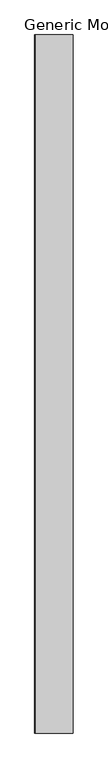
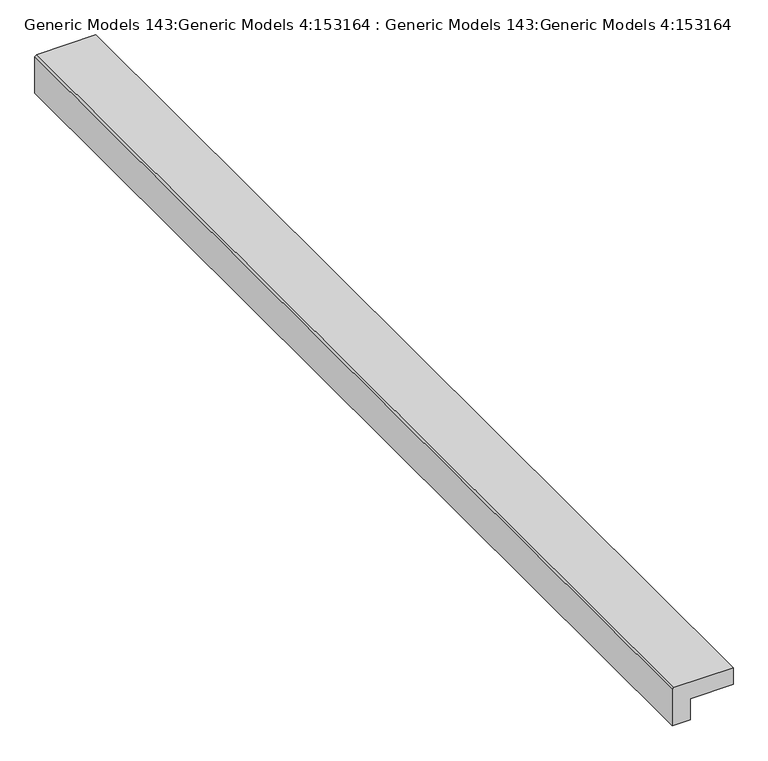
"""IFC4 building model written with IfcOpenShell, lengths in millimetres: proxy geometry, Generic Models 143:Generic Models 4:153164 : Generic Models 143:Generic Models 4:153164."""

from ifc_helpers import new_model, si_unit, frame, origin, place, context, project, spatial, polyline, outline, extrude, source, transform, mapped, element, save


def generic_models_143_generic_models_4_153164_generic_models_44f4f31f(model_context):
    return source(origin(), model_context, "Body", "SweptSolid", [
        extrude(outline(polyline([(-38.1, -6651.746787), (-57.15, -6670.796787), (-495.3, -6670.796787), (-495.3, -6467.596787), (-241.3, -6467.596787), (-241.3, -5978.646787), (-38.1, -5978.646787), (-38.1, -6651.746787)])), frame((0.0, -5303.1974793, 0.0), z_axis=(0.0, 1.0, 0.0), x_axis=(0.0, 0.0, 1.0)), (0.0, 0.0, 1.0), 12547.6),
    ])


if __name__ == "__main__":
    model = new_model("IFC4")
    model_context = context("Model", 3, world=origin())
    ifc_project = project(units=[si_unit("LENGTHUNIT", "METRE", prefix="MILLI")], contexts=[model_context])
    site = spatial("IfcSite", under=ifc_project)
    building = spatial("IfcBuilding", under=site)
    placement = place(None, origin())
    generic_models_143_generic_models_4_153164_generic_models_shape = generic_models_143_generic_models_4_153164_generic_models_44f4f31f(model_context)
    element("IfcBuildingElementProxy", 1, Name="Generic Models 143:Generic Models 4:153164 : Generic Models 143:Generic Models 4:153164", ObjectType="Generic Models 143:Generic Models 4:153164 : Generic Models 143:Generic Models 4:153164", at=placement, inside=building, context=model_context, shape_type="MappedRepresentation", body=[
        mapped(generic_models_143_generic_models_4_153164_generic_models_shape, transform((0.0, 0.0, 0.0), x_axis=(1.0, 0.0, 0.0), y_axis=(0.0, 1.0, 0.0), z_axis=(0.0, 0.0, 1.0))),
    ])
    save(model, "model.ifc")

# Revit data of these elements
# Type "Generic Models 143:Generic Models 4:153164 : Generic Models 143:Generic Models 4:153164"
#   NameOverride = "Generic Models 143:Generic Models 4:153164"
#   ObjectTypeOverride = "Generic Models 143:Generic Models 4"
#   Reference = "Generic Models 4"
#   Category = "Generic Models"
#   Tag = "153164"
# Element 1 (IfcBuildingElementProxy, "Generic Models 143:Generic Models 4:153164 : Generic Models 143:Generic Models 4:153164")
#   Materials on its faces: "_ 8\" CONCRETE SLAB W/ GRADE BEAM (SEE STRUCT. DWGS) 10051"
# Materials
#   "_ 8\" CONCRETE SLAB W/ GRADE BEAM (SEE STRUCT. DWGS) 10051": class "Unassigned", colour RGB 191 191 191, transparency 0
